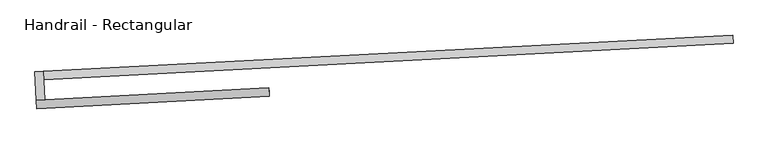
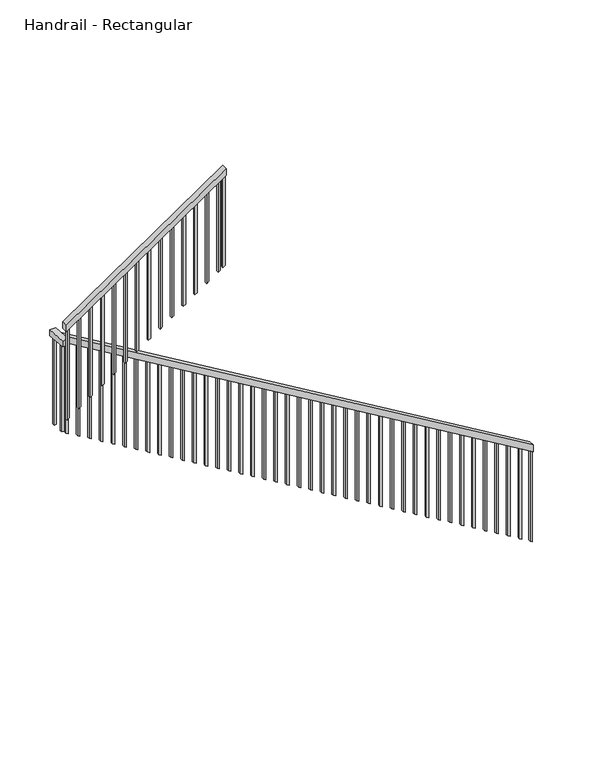
"""IFC4 building model written with IfcOpenShell, lengths in millimetres: railing geometry, Handrail - Rectangular."""

import ifcopenshell
import ifcopenshell.guid

model = None  # the IFC model being written
_history = None  # IfcOwnerHistory: only IFC2X3 demands one
_inside = {}  # id of a spatial element -> (the spatial element, [elements in it])
_under = {}  # id of a project, library or spatial element -> (it, [spatial elements below it])
_declared = {}  # id of a project -> (the project, [libraries it declares])
_typed = {}  # id of a type object -> (the type object, [elements of that type])
_made_of = {}  # id of a material, layer set ... -> (it, [elements and type objects made of it])


def new_model(schema):
    """Start an empty IFC model of exactly this schema.

    Asked for "IFC4X3", IfcOpenShell would pick the latest addendum, in which some entities
    have other attributes; the version numbers below select the first issue.
    IFC2X3 requires an IfcOwnerHistory on every rooted entity: one is made here for all.
    """
    global model, _history
    if schema == "IFC4X3":
        model = ifcopenshell.file(schema_version=(4, 3, 0, 0))
    else:
        model = ifcopenshell.file(schema=schema)
    _inside.clear()
    _under.clear()
    _declared.clear()
    _typed.clear()
    _made_of.clear()
    _history = None
    if model.schema == "IFC2X3":
        org = make("IfcOrganization", Name="unknown")
        user = make(
            "IfcPersonAndOrganization",
            ThePerson=make("IfcPerson", FamilyName="unknown"),
            TheOrganization=org,
        )
        app = make(
            "IfcApplication",
            ApplicationDeveloper=org,
            Version="unknown",
            ApplicationFullName="unknown",
            ApplicationIdentifier="unknown",
        )
        _history = make(
            "IfcOwnerHistory",
            OwningUser=user,
            OwningApplication=app,
            ChangeAction="ADDED",
            CreationDate=0,
        )
    return model


def make(cls, **values):
    """One entity of the class cls with the attributes given. An attribute that is None is left unset."""
    return model.create_entity(
        cls, **{name: value for name, value in values.items() if value is not None}
    )


def rooted(cls, **values):
    """An entity with a GlobalId (a new one), such as an element, a storey or a relation."""
    return make(cls, GlobalId=ifcopenshell.guid.new(), OwnerHistory=_history, **values)


def si_unit(unit_type, name, prefix=None):
    """IfcSIUnit, for example si_unit("LENGTHUNIT", "METRE", prefix="MILLI")."""
    return make("IfcSIUnit", UnitType=unit_type, Prefix=prefix, Name=name)


def assignment(units):
    """IfcUnitAssignment: the units of a project."""
    return None if units is None else make("IfcUnitAssignment", Units=units)


def point(xyz):
    """IfcCartesianPoint."""
    return None if xyz is None else make("IfcCartesianPoint", Coordinates=xyz)


def direction(xyz):
    """IfcDirection."""
    return None if xyz is None else make("IfcDirection", DirectionRatios=xyz)


def frame(location, z_axis=None, x_axis=None):
    """IfcAxis2Placement3D, a coordinate frame: its origin and axes. An axis left out is left unset."""
    return make(
        "IfcAxis2Placement3D",
        Location=point(location),
        Axis=direction(z_axis),
        RefDirection=direction(x_axis),
    )


def origin():
    """The frame at (0, 0, 0) with its axes left unset."""
    return frame((0.0, 0.0, 0.0))


def place(relative_to, where):
    """IfcLocalPlacement: puts the frame where relative to a parent placement (None: the world)."""
    return make(
        "IfcLocalPlacement", PlacementRelTo=relative_to, RelativePlacement=where
    )


def context(
    kind, dimensions, precision=None, world=None, true_north=None, identifier=None
):
    """IfcGeometricRepresentationContext, for example the 3D "Model" context."""
    return make(
        "IfcGeometricRepresentationContext",
        ContextIdentifier=identifier,
        ContextType=kind,
        CoordinateSpaceDimension=dimensions,
        Precision=precision,
        WorldCoordinateSystem=world,
        TrueNorth=true_north,
    )


def project(units=None, contexts=None):
    """IfcProject with its units and contexts."""
    return rooted(
        "IfcProject",
        Name="project",
        RepresentationContexts=contexts,
        UnitsInContext=assignment(units),
    )


def spatial(cls, under=None, at=None, **own):
    """A site, building, storey or space (cls), placed at a placement, below another one or the project."""
    s = rooted(cls, ObjectPlacement=at, **own)
    if under is not None:
        _under.setdefault(under.id(), (under, []))[1].append(s)
    return s


def polyline(points):
    """IfcPolyline through the points."""
    return make("IfcPolyline", Points=[point(p) for p in points])


def outline(outer, holes=None, kind="AREA"):
    """IfcArbitraryClosedProfileDef: a profile drawn as a closed curve; with holes, ...WithVoids."""
    if holes is None:
        return make("IfcArbitraryClosedProfileDef", ProfileType=kind, OuterCurve=outer)
    return make(
        "IfcArbitraryProfileDefWithVoids",
        ProfileType=kind,
        OuterCurve=outer,
        InnerCurves=holes,
    )


def extrude(swept, where, along, depth):
    """IfcExtrudedAreaSolid: the profile swept, set in the frame where, extruded along a direction by depth."""
    return make(
        "IfcExtrudedAreaSolid",
        SweptArea=swept,
        Position=where,
        ExtrudedDirection=direction(along),
        Depth=depth,
    )


def shape(context_of_items, identifier, shape_type, items):
    """IfcShapeRepresentation: the items that make up one representation, for example the "Body"."""
    return make(
        "IfcShapeRepresentation",
        ContextOfItems=context_of_items,
        RepresentationIdentifier=identifier,
        RepresentationType=shape_type,
        Items=items,
    )


def source(mapping_origin, context_of_items, identifier, shape_type, items):
    """IfcRepresentationMap: a shape defined once, which mapped items show again and again."""
    return make(
        "IfcRepresentationMap",
        MappingOrigin=mapping_origin,
        MappedRepresentation=shape(context_of_items, identifier, shape_type, items),
    )


def transform(
    local_origin,
    x_axis=None,
    y_axis=None,
    z_axis=None,
    scale=None,
    scale2=None,
    scale3=None,
    uniform=True,
):
    """IfcCartesianTransformationOperator3D, or its non-uniform kind. x_axis, y_axis, z_axis: its Axis1, 2, 3."""
    if uniform:
        return make(
            "IfcCartesianTransformationOperator3D",
            Axis1=direction(x_axis),
            Axis2=direction(y_axis),
            LocalOrigin=point(local_origin),
            Scale=scale,
            Axis3=direction(z_axis),
        )
    return make(
        "IfcCartesianTransformationOperator3DnonUniform",
        Axis1=direction(x_axis),
        Axis2=direction(y_axis),
        LocalOrigin=point(local_origin),
        Scale=scale,
        Axis3=direction(z_axis),
        Scale2=scale2,
        Scale3=scale3,
    )


def mapped(mapping_source, mapping_target):
    """IfcMappedItem: shows the shape of a source again, moved by a transform."""
    return make(
        "IfcMappedItem", MappingSource=mapping_source, MappingTarget=mapping_target
    )


def made_of(thing, what):
    """Note that an element or type object is made of a material, layer set ...; save() writes the relation."""
    if what is not None:
        _made_of.setdefault(what.id(), (what, []))[1].append(thing)
    return thing


def element(
    cls,
    number,
    at=None,
    inside=None,
    cuts=None,
    type_object=None,
    material=None,
    context=None,
    identifier="Body",
    shape_type=None,
    held_by="IfcProductDefinitionShape",
    body=None,
    shapes=None,
    **own,
):
    """One element of the class cls, such as IfcWall. Its Tag is "e" and its number.

    at: its placement. inside: the storey or other place that contains it. cuts: it is an
    opening in that element (IfcRelVoidsElement). A single representation is given by context,
    identifier, shape_type and body (its items); several are given by shapes. held_by: the class
    of the entity that holds the representations. save() writes the other relations.
    """
    e = rooted(cls, Tag="e%d" % number, ObjectPlacement=at, **own)
    if body is not None:
        shapes = [shape(context, identifier, shape_type, body)]
    if shapes is not None:
        e.Representation = make(held_by, Representations=shapes)
    if inside is not None:
        _inside.setdefault(inside.id(), (inside, []))[1].append(e)
    if cuts is not None:
        rooted(
            "IfcRelVoidsElement", RelatingBuildingElement=cuts, RelatedOpeningElement=e
        )
    if type_object is not None:
        _typed.setdefault(type_object.id(), (type_object, []))[1].append(e)
    return made_of(e, material)


def aggregate(whole, parts):
    """IfcRelAggregates: a whole, such as a stair, and the parts it consists of."""
    return rooted("IfcRelAggregates", RelatingObject=whole, RelatedObjects=parts)


def save(model, path):
    """Write the relations noted so far, then the file.

    IfcRelAggregates (storeys below a building ...), IfcRelContainedInSpatialStructure (elements
    in a storey), IfcRelDefinesByType, IfcRelAssociatesMaterial and IfcRelDeclares: one each for
    every whole, place, type object, material and project.
    """
    for whole, parts in _under.values():
        aggregate(whole, parts)
    for where, things in _inside.values():
        rooted(
            "IfcRelContainedInSpatialStructure",
            RelatedElements=things,
            RelatingStructure=where,
        )
    for kind, things in _typed.values():
        rooted("IfcRelDefinesByType", RelatedObjects=things, RelatingType=kind)
    for what, things in _made_of.values():
        rooted("IfcRelAssociatesMaterial", RelatedObjects=things, RelatingMaterial=what)
    for by, libraries in _declared.values():
        rooted("IfcRelDeclares", RelatingContext=by, RelatedDefinitions=libraries)
    model.write(path)


def handrail_rectangular_b2c7f8ce(model_context):
    return source(origin(), model_context, "Body", "SweptSolid", [
        extrude(outline(polyline([(-31.4876033, -50.8), (0.0, 0.0), (4871.0206406, 0.0), (4839.5330373, -50.8), (-31.4876033, -50.8)])), frame((12083.9919851, -25001.0309623, 1087.5818182), z_axis=(-0.05233595624293972, 0.9986295347545743, 0.0), x_axis=(-0.8488007555029385, -0.04448376264967305, 0.5268381841876767)), (0.0, 0.0, 1.0), 50.8),
        extrude(outline(polyline([(7896.0769384, -25169.6405746), (7946.8073187, -25166.981908), (7955.7803184, -25338.1969417), (7905.0499381, -25340.8556083), (7896.0769384, -25169.6405746)])), frame((0.0, 0.0, 3634.5090909), z_axis=(0.0, 0.0, 1.0), x_axis=(1.0, 0.0, 0.0)), (0.0, 0.0, 1.0), 50.8),
        extrude(outline(polyline([(31.4876033, -50.8), (0.0, 0.0), (1643.5959216, 0.0), (1675.0835249, -50.8), (31.4876033, -50.8)])), frame((7907.7086047, -25391.5859887, 3798.7237847), z_axis=(-0.052335956242938755, 0.9986295347545742, 0.0), x_axis=(0.8488007555029388, 0.044483762649671764, 0.5268381841876766)), (0.0, 0.0, 1.0), 50.8),
        extrude(outline(polyline([(234.5039256, 19.0500001), (1048.9045305, 19.0500001), (1037.0966792, 0.0), (222.6960744, 0.0), (234.5039256, 19.0500001)])), frame((9260.7447974, -25304.7795805, 4861.7452723), z_axis=(-0.052335956242940136, 0.9986295347545743, 0.0), x_axis=(0.0, 0.0, -1.0)), (0.0, 0.0, 1.0), 19.05),
        extrude(outline(polyline([(234.5039257, 19.05), (1048.9045305, 19.05), (1037.0966792, 0.0), (222.6960744, 0.0), (234.5039257, 19.05)])), frame((9159.2840366, -25310.0969137, 4798.7700657), z_axis=(-0.052335956242940136, 0.9986295347545743, 0.0), x_axis=(0.0, 0.0, -1.0)), (0.0, 0.0, 1.0), 19.05),
        extrude(outline(polyline([(234.5039256, 19.05), (1048.9045304, 19.05), (1037.0966791, 0.0), (222.6960743, 0.0), (234.5039256, 19.05)])), frame((9057.8232759, -25315.4142468, 4735.794859), z_axis=(-0.052335956242940136, 0.9986295347545743, 0.0), x_axis=(0.0, 0.0, -1.0)), (0.0, 0.0, 1.0), 19.05),
        extrude(outline(polyline([(234.5039256, 19.0500001), (1048.9045304, 19.0500001), (1037.0966792, 0.0), (222.6960743, 0.0), (234.5039256, 19.0500001)])), frame((8956.3625152, -25320.73158, 4672.8196524), z_axis=(-0.052335956242940136, 0.9986295347545743, 0.0), x_axis=(0.0, 0.0, -1.0)), (0.0, 0.0, 1.0), 19.05),
        extrude(outline(polyline([(234.5039256, 19.05), (1048.9045304, 19.05), (1037.0966792, 0.0), (222.6960744, 0.0), (234.5039256, 19.05)])), frame((8854.9017544, -25326.0489131, 4609.8444458), z_axis=(-0.052335956242940136, 0.9986295347545743, 0.0), x_axis=(0.0, 0.0, -1.0)), (0.0, 0.0, 1.0), 19.05),
        extrude(outline(polyline([(234.5039256, 19.05), (1048.9045304, 19.05), (1037.0966792, 0.0), (222.6960744, 0.0), (234.5039256, 19.05)])), frame((8753.4409937, -25331.3662463, 4546.8692392), z_axis=(-0.052335956242940136, 0.9986295347545743, 0.0), x_axis=(0.0, 0.0, -1.0)), (0.0, 0.0, 1.0), 19.05),
        extrude(outline(polyline([(234.5039256, 19.0500001), (1048.9045304, 19.0500001), (1037.0966792, 0.0), (222.6960744, 0.0), (234.5039256, 19.0500001)])), frame((8651.980233, -25336.6835795, 4483.8940326), z_axis=(-0.052335956242940136, 0.9986295347545743, 0.0), x_axis=(0.0, 0.0, -1.0)), (0.0, 0.0, 1.0), 19.05),
        extrude(outline(polyline([(234.5039256, 19.05), (1048.9045304, 19.05), (1037.0966792, 0.0), (222.6960744, 0.0), (234.5039256, 19.05)])), frame((8550.5194722, -25342.0009126, 4420.918826), z_axis=(-0.052335956242940136, 0.9986295347545743, 0.0), x_axis=(0.0, 0.0, -1.0)), (0.0, 0.0, 1.0), 19.05),
        extrude(outline(polyline([(234.5039256, 19.05), (1048.9045305, 19.05), (1037.0966792, 0.0), (222.6960744, 0.0), (234.5039256, 19.05)])), frame((8449.0587115, -25347.3182458, 4357.9436194), z_axis=(-0.052335956242940136, 0.9986295347545743, 0.0), x_axis=(0.0, 0.0, -1.0)), (0.0, 0.0, 1.0), 19.05),
        extrude(outline(polyline([(234.5039257, 19.0500001), (1048.9045305, 19.0500001), (1037.0966792, 0.0), (222.6960744, 0.0), (234.5039257, 19.0500001)])), frame((8347.5979508, -25352.6355789, 4294.9684128), z_axis=(-0.052335956242940136, 0.9986295347545743, 0.0), x_axis=(0.0, 0.0, -1.0)), (0.0, 0.0, 1.0), 19.05),
        extrude(outline(polyline([(234.5039257, 19.05), (1048.9045305, 19.05), (1037.0966792, 0.0), (222.6960744, 0.0), (234.5039257, 19.05)])), frame((8246.13719, -25357.9529121, 4231.9932062), z_axis=(-0.052335956242940136, 0.9986295347545743, 0.0), x_axis=(0.0, 0.0, -1.0)), (0.0, 0.0, 1.0), 19.05),
        extrude(outline(polyline([(234.5039256, 19.05), (1048.9045304, 19.05), (1037.0966791, 0.0), (222.6960743, 0.0), (234.5039256, 19.05)])), frame((8144.6764293, -25363.2702452, 4169.0179995), z_axis=(-0.052335956242940136, 0.9986295347545743, 0.0), x_axis=(0.0, 0.0, -1.0)), (0.0, 0.0, 1.0), 19.05),
        extrude(outline(polyline([(234.5039256, 19.0500001), (1048.9045304, 19.0500001), (1037.0966792, 0.0), (222.6960743, 0.0), (234.5039256, 19.0500001)])), frame((8043.2156686, -25368.5875784, 4106.0427929), z_axis=(-0.052335956242940136, 0.9986295347545743, 0.0), x_axis=(0.0, 0.0, -1.0)), (0.0, 0.0, 1.0), 19.05),
        extrude(outline(polyline([(7937.1022413, -25285.1267459), (7938.0992413, -25304.1506385), (7919.0753487, -25305.1476385), (7918.0783487, -25286.1237459), (7937.1022413, -25285.1267459)])), frame((0.0, 0.0, 2847.1090909), z_axis=(0.0, 0.0, 1.0), x_axis=(1.0, 0.0, 0.0)), (0.0, 0.0, 1.0), 787.4),
        extrude(outline(polyline([(222.6960744, 19.0500001), (1037.0966792, 19.0500001), (1048.9045304, 0.0), (234.5039256, 0.0), (222.6960744, 19.0500001)])), frame((8034.2426689, -25197.3725446, 3775.4229582), z_axis=(-0.05233595624293971, 0.9986295347545743, 0.0), x_axis=(0.0, 0.0, -1.0)), (0.0, 0.0, 1.0), 19.05),
        extrude(outline(polyline([(222.6960744, 19.05), (1037.0966792, 19.05), (1048.9045304, 0.0), (234.5039256, 0.0), (222.6960744, 19.05)])), frame((8135.7034296, -25192.0552115, 3712.4477516), z_axis=(-0.05233595624293971, 0.9986295347545743, 0.0), x_axis=(0.0, 0.0, -1.0)), (0.0, 0.0, 1.0), 19.05),
        extrude(outline(polyline([(222.6960744, 19.05), (1037.0966792, 19.05), (1048.9045304, 0.0), (234.5039256, 0.0), (222.6960744, 19.05)])), frame((8237.1641903, -25186.7378783, 3649.472545), z_axis=(-0.05233595624293971, 0.9986295347545743, 0.0), x_axis=(0.0, 0.0, -1.0)), (0.0, 0.0, 1.0), 19.05),
        extrude(outline(polyline([(222.6960744, 19.0500001), (1037.0966792, 19.0500001), (1048.9045304, 0.0), (234.5039256, 0.0), (222.6960744, 19.0500001)])), frame((8338.6249511, -25181.4205452, 3586.4973384), z_axis=(-0.05233595624293971, 0.9986295347545743, 0.0), x_axis=(0.0, 0.0, -1.0)), (0.0, 0.0, 1.0), 19.05),
        extrude(outline(polyline([(222.6960744, 19.05), (1037.0966792, 19.05), (1048.9045305, 0.0), (234.5039256, 0.0), (222.6960744, 19.05)])), frame((8440.0857118, -25176.103212, 3523.5221318), z_axis=(-0.05233595624293971, 0.9986295347545743, 0.0), x_axis=(0.0, 0.0, -1.0)), (0.0, 0.0, 1.0), 19.05),
        extrude(outline(polyline([(222.6960744, 19.05), (1037.0966792, 19.05), (1048.9045305, 0.0), (234.5039257, 0.0), (222.6960744, 19.05)])), frame((8541.5464725, -25170.7858789, 3460.5469252), z_axis=(-0.05233595624293971, 0.9986295347545743, 0.0), x_axis=(0.0, 0.0, -1.0)), (0.0, 0.0, 1.0), 19.05),
        extrude(outline(polyline([(222.6960744, 19.0500001), (1037.0966792, 19.0500001), (1048.9045305, 0.0), (234.5039257, 0.0), (222.6960744, 19.0500001)])), frame((8643.0072333, -25165.4685457, 3397.5717186), z_axis=(-0.05233595624293971, 0.9986295347545743, 0.0), x_axis=(0.0, 0.0, -1.0)), (0.0, 0.0, 1.0), 19.05),
        extrude(outline(polyline([(222.6960743, 19.05), (1037.0966791, 19.05), (1048.9045304, 0.0), (234.5039256, 0.0), (222.6960743, 19.05)])), frame((8744.467994, -25160.1512126, 3334.5965119), z_axis=(-0.05233595624293971, 0.9986295347545743, 0.0), x_axis=(0.0, 0.0, -1.0)), (0.0, 0.0, 1.0), 19.05),
        extrude(outline(polyline([(222.6960744, 19.05), (1037.0966792, 19.05), (1048.9045304, 0.0), (234.5039256, 0.0), (222.6960744, 19.05)])), frame((8845.9287547, -25154.8338794, 3271.6213053), z_axis=(-0.05233595624293971, 0.9986295347545743, 0.0), x_axis=(0.0, 0.0, -1.0)), (0.0, 0.0, 1.0), 19.05),
        extrude(outline(polyline([(222.6960744, 19.0500001), (1037.0966792, 19.0500001), (1048.9045304, 0.0), (234.5039256, 0.0), (222.6960744, 19.0500001)])), frame((8947.3895155, -25149.5165463, 3208.6460987), z_axis=(-0.05233595624293971, 0.9986295347545743, 0.0), x_axis=(0.0, 0.0, -1.0)), (0.0, 0.0, 1.0), 19.05),
        extrude(outline(polyline([(222.6960744, 19.05), (1037.0966792, 19.05), (1048.9045304, 0.0), (234.5039256, 0.0), (222.6960744, 19.05)])), frame((9048.8502762, -25144.1992131, 3145.6708921), z_axis=(-0.05233595624293971, 0.9986295347545743, 0.0), x_axis=(0.0, 0.0, -1.0)), (0.0, 0.0, 1.0), 19.05),
        extrude(outline(polyline([(222.6960744, 19.05), (1037.0966792, 19.05), (1048.9045304, 0.0), (234.5039256, 0.0), (222.6960744, 19.05)])), frame((9150.3110369, -25138.8818799, 3082.6956855), z_axis=(-0.05233595624293971, 0.9986295347545743, 0.0), x_axis=(0.0, 0.0, -1.0)), (0.0, 0.0, 1.0), 19.05),
        extrude(outline(polyline([(222.6960744, 19.0500001), (1037.0966792, 19.0500001), (1048.9045304, 0.0), (234.5039256, 0.0), (222.6960744, 19.0500001)])), frame((9251.7717977, -25133.5645468, 3019.7204789), z_axis=(-0.05233595624293971, 0.9986295347545743, 0.0), x_axis=(0.0, 0.0, -1.0)), (0.0, 0.0, 1.0), 19.05),
        extrude(outline(polyline([(222.6960744, 19.05), (1037.0966792, 19.05), (1048.9045305, 0.0), (234.5039256, 0.0), (222.6960744, 19.05)])), frame((9353.2325584, -25128.2472136, 2956.7452723), z_axis=(-0.05233595624293971, 0.9986295347545743, 0.0), x_axis=(0.0, 0.0, -1.0)), (0.0, 0.0, 1.0), 19.05),
        extrude(outline(polyline([(222.6960744, 19.05), (1037.0966792, 19.05), (1048.9045305, 0.0), (234.5039257, 0.0), (222.6960744, 19.05)])), frame((9454.6933191, -25122.9298805, 2893.7700657), z_axis=(-0.05233595624293971, 0.9986295347545743, 0.0), x_axis=(0.0, 0.0, -1.0)), (0.0, 0.0, 1.0), 19.05),
        extrude(outline(polyline([(222.6960743, 19.05), (1037.0966791, 19.05), (1048.9045304, 0.0), (234.5039256, 0.0), (222.6960743, 19.05)])), frame((9556.1540798, -25117.6125473, 2830.794859), z_axis=(-0.05233595624293971, 0.9986295347545743, 0.0), x_axis=(0.0, 0.0, -1.0)), (0.0, 0.0, 1.0), 19.05),
        extrude(outline(polyline([(222.6960743, 19.0500001), (1037.0966792, 19.0500001), (1048.9045304, 0.0), (234.5039256, 0.0), (222.6960743, 19.0500001)])), frame((9657.6148406, -25112.2952142, 2767.8196524), z_axis=(-0.05233595624293971, 0.9986295347545743, 0.0), x_axis=(0.0, 0.0, -1.0)), (0.0, 0.0, 1.0), 19.05),
        extrude(outline(polyline([(222.6960744, 19.05), (1037.0966792, 19.05), (1048.9045304, 0.0), (234.5039256, 0.0), (222.6960744, 19.05)])), frame((9759.0756013, -25106.977881, 2704.8444458), z_axis=(-0.05233595624293971, 0.9986295347545743, 0.0), x_axis=(0.0, 0.0, -1.0)), (0.0, 0.0, 1.0), 19.05),
        extrude(outline(polyline([(222.6960744, 19.05), (1037.0966792, 19.05), (1048.9045304, 0.0), (234.5039256, 0.0), (222.6960744, 19.05)])), frame((9860.536362, -25101.6605479, 2641.8692392), z_axis=(-0.05233595624293971, 0.9986295347545743, 0.0), x_axis=(0.0, 0.0, -1.0)), (0.0, 0.0, 1.0), 19.05),
        extrude(outline(polyline([(222.6960744, 19.0500001), (1037.0966792, 19.0500001), (1048.9045304, 0.0), (234.5039256, 0.0), (222.6960744, 19.0500001)])), frame((9961.9971228, -25096.3432147, 2578.8940326), z_axis=(-0.05233595624293971, 0.9986295347545743, 0.0), x_axis=(0.0, 0.0, -1.0)), (0.0, 0.0, 1.0), 19.05),
        extrude(outline(polyline([(222.6960744, 19.05), (1037.0966792, 19.05), (1048.9045304, 0.0), (234.5039256, 0.0), (222.6960744, 19.05)])), frame((10063.4578835, -25091.0258816, 2515.918826), z_axis=(-0.05233595624293971, 0.9986295347545743, 0.0), x_axis=(0.0, 0.0, -1.0)), (0.0, 0.0, 1.0), 19.05),
        extrude(outline(polyline([(222.6960744, 19.05), (1037.0966792, 19.05), (1048.9045305, 0.0), (234.5039256, 0.0), (222.6960744, 19.05)])), frame((10164.9186442, -25085.7085484, 2452.9436194), z_axis=(-0.05233595624293971, 0.9986295347545743, 0.0), x_axis=(0.0, 0.0, -1.0)), (0.0, 0.0, 1.0), 19.05),
        extrude(outline(polyline([(222.6960744, 19.0500001), (1037.0966792, 19.0500001), (1048.9045305, 0.0), (234.5039257, 0.0), (222.6960744, 19.0500001)])), frame((10266.379405, -25080.3912153, 2389.9684128), z_axis=(-0.05233595624293971, 0.9986295347545743, 0.0), x_axis=(0.0, 0.0, -1.0)), (0.0, 0.0, 1.0), 19.05),
        extrude(outline(polyline([(222.6960744, 19.05), (1037.0966792, 19.05), (1048.9045305, 0.0), (234.5039257, 0.0), (222.6960744, 19.05)])), frame((10367.8401657, -25075.0738821, 2326.9932062), z_axis=(-0.05233595624293971, 0.9986295347545743, 0.0), x_axis=(0.0, 0.0, -1.0)), (0.0, 0.0, 1.0), 19.05),
        extrude(outline(polyline([(222.6960743, 19.05), (1037.0966791, 19.05), (1048.9045304, 0.0), (234.5039256, 0.0), (222.6960743, 19.05)])), frame((10469.3009264, -25069.7565489, 2264.0179995), z_axis=(-0.05233595624293971, 0.9986295347545743, 0.0), x_axis=(0.0, 0.0, -1.0)), (0.0, 0.0, 1.0), 19.05),
        extrude(outline(polyline([(222.6960743, 19.0500001), (1037.0966792, 19.0500001), (1048.9045304, 0.0), (234.5039256, 0.0), (222.6960743, 19.0500001)])), frame((10570.7616872, -25064.4392158, 2201.0427929), z_axis=(-0.05233595624293971, 0.9986295347545743, 0.0), x_axis=(0.0, 0.0, -1.0)), (0.0, 0.0, 1.0), 19.05),
        extrude(outline(polyline([(222.6960744, 19.05), (1037.0966792, 19.05), (1048.9045304, 0.0), (234.5039256, 0.0), (222.6960744, 19.05)])), frame((10672.2224479, -25059.1218826, 2138.0675863), z_axis=(-0.05233595624293971, 0.9986295347545743, 0.0), x_axis=(0.0, 0.0, -1.0)), (0.0, 0.0, 1.0), 19.05),
        extrude(outline(polyline([(222.6960744, 19.05), (1037.0966792, 19.05), (1048.9045304, 0.0), (234.5039256, 0.0), (222.6960744, 19.05)])), frame((10773.6832086, -25053.8045495, 2075.0923797), z_axis=(-0.05233595624293971, 0.9986295347545743, 0.0), x_axis=(0.0, 0.0, -1.0)), (0.0, 0.0, 1.0), 19.05),
        extrude(outline(polyline([(222.6960744, 19.0500001), (1037.0966792, 19.0500001), (1048.9045304, 0.0), (234.5039256, 0.0), (222.6960744, 19.0500001)])), frame((10875.1439694, -25048.4872163, 2012.1171731), z_axis=(-0.05233595624293971, 0.9986295347545743, 0.0), x_axis=(0.0, 0.0, -1.0)), (0.0, 0.0, 1.0), 19.05),
        extrude(outline(polyline([(222.6960744, 19.0500001), (1037.0966792, 19.0500001), (1048.9045304, 0.0), (234.5039256, 0.0), (222.6960744, 19.0500001)])), frame((10976.6047301, -25043.1698832, 1949.1419665), z_axis=(-0.05233595624293971, 0.9986295347545743, 0.0), x_axis=(0.0, 0.0, -1.0)), (0.0, 0.0, 1.0), 19.05),
        extrude(outline(polyline([(222.6960744, 19.05), (1037.0966792, 19.05), (1048.9045305, 0.0), (234.5039256, 0.0), (222.6960744, 19.05)])), frame((11078.0654908, -25037.85255, 1886.1667599), z_axis=(-0.05233595624293971, 0.9986295347545743, 0.0), x_axis=(0.0, 0.0, -1.0)), (0.0, 0.0, 1.0), 19.05),
        extrude(outline(polyline([(222.6960744, 19.05), (1037.0966792, 19.05), (1048.9045305, 0.0), (234.5039257, 0.0), (222.6960744, 19.05)])), frame((11179.5262515, -25032.5352169, 1823.1915533), z_axis=(-0.05233595624293971, 0.9986295347545743, 0.0), x_axis=(0.0, 0.0, -1.0)), (0.0, 0.0, 1.0), 19.05),
        extrude(outline(polyline([(222.6960744, 19.0500001), (1037.0966792, 19.0500001), (1048.9045305, 0.0), (234.5039257, 0.0), (222.6960744, 19.0500001)])), frame((11280.9870123, -25027.2178837, 1760.2163467), z_axis=(-0.05233595624293971, 0.9986295347545743, 0.0), x_axis=(0.0, 0.0, -1.0)), (0.0, 0.0, 1.0), 19.05),
        extrude(outline(polyline([(222.6960743, 19.05), (1037.0966792, 19.05), (1048.9045304, 0.0), (234.5039256, 0.0), (222.6960743, 19.05)])), frame((11382.447773, -25021.9005506, 1697.24114), z_axis=(-0.05233595624293971, 0.9986295347545743, 0.0), x_axis=(0.0, 0.0, -1.0)), (0.0, 0.0, 1.0), 19.05),
        extrude(outline(polyline([(222.6960744, 19.05), (1037.0966792, 19.05), (1048.9045304, 0.0), (234.5039256, 0.0), (222.6960744, 19.05)])), frame((11483.9085337, -25016.5832174, 1634.2659334), z_axis=(-0.05233595624293971, 0.9986295347545743, 0.0), x_axis=(0.0, 0.0, -1.0)), (0.0, 0.0, 1.0), 19.05),
        extrude(outline(polyline([(222.6960744, 19.0500001), (1037.0966792, 19.0500001), (1048.9045304, 0.0), (234.5039256, 0.0), (222.6960744, 19.0500001)])), frame((11585.3692945, -25011.2658842, 1571.2907268), z_axis=(-0.05233595624293971, 0.9986295347545743, 0.0), x_axis=(0.0, 0.0, -1.0)), (0.0, 0.0, 1.0), 19.05),
        extrude(outline(polyline([(222.6960744, 19.05), (1037.0966792, 19.05), (1048.9045304, 0.0), (234.5039256, 0.0), (222.6960744, 19.05)])), frame((11686.8300552, -25005.9485511, 1508.3155202), z_axis=(-0.05233595624293971, 0.9986295347545743, 0.0), x_axis=(0.0, 0.0, -1.0)), (0.0, 0.0, 1.0), 19.05),
        extrude(outline(polyline([(222.6960744, 19.05), (1037.0966792, 19.05), (1048.9045304, 0.0), (234.5039256, 0.0), (222.6960744, 19.05)])), frame((11788.2908159, -25000.6312179, 1445.3403136), z_axis=(-0.05233595624293971, 0.9986295347545743, 0.0), x_axis=(0.0, 0.0, -1.0)), (0.0, 0.0, 1.0), 19.05),
        extrude(outline(polyline([(222.6960744, 19.0500001), (1037.0966792, 19.0500001), (1048.9045304, 0.0), (234.5039256, 0.0), (222.6960744, 19.0500001)])), frame((11889.7515767, -24995.3138848, 1382.365107), z_axis=(-0.05233595624293971, 0.9986295347545743, 0.0), x_axis=(0.0, 0.0, -1.0)), (0.0, 0.0, 1.0), 19.05),
        extrude(outline(polyline([(222.6960744, 19.05), (1037.0966792, 19.05), (1048.9045305, 0.0), (234.5039257, 0.0), (222.6960744, 19.05)])), frame((11991.2123374, -24989.9965516, 1319.3899004), z_axis=(-0.05233595624293971, 0.9986295347545743, 0.0), x_axis=(0.0, 0.0, -1.0)), (0.0, 0.0, 1.0), 19.05),
        extrude(outline(polyline([(234.5039256, 19.0500001), (1048.9045304, 19.0500001), (1037.0966792, 0.0), (222.6960744, 0.0), (234.5039256, 19.0500001)])), frame((7941.7549079, -25373.9049115, 4043.0675863), z_axis=(-0.052335956242940136, 0.9986295347545743, 0.0), x_axis=(0.0, 0.0, -1.0)), (0.0, 0.0, 1.0), 19.05),
        extrude(outline(polyline([(7931.7849082, -25183.6659852), (7932.7819082, -25202.6898778), (7913.7580155, -25203.6868778), (7912.7610155, -25184.6629851), (7931.7849082, -25183.6659852)])), frame((0.0, 0.0, 2847.1090909), z_axis=(0.0, 0.0, 1.0), x_axis=(1.0, 0.0, 0.0)), (0.0, 0.0, 1.0), 787.4),
        extrude(outline(polyline([(234.5039257, 19.05), (1048.9045305, 19.05), (1037.0966792, 0.0), (222.6960744, 0.0), (234.5039257, 19.05)])), frame((9301.9632314, -25302.6194139, 4887.32895), z_axis=(-0.052335956242940136, 0.9986295347545743, 0.0), x_axis=(0.0, 0.0, -1.0)), (0.0, 0.0, 1.0), 19.05),
        extrude(outline(polyline([(222.6960744, 19.05), (1037.0966792, 19.05), (1048.9045305, 0.0), (234.5039256, 0.0), (222.6960744, 19.05)])), frame((12083.1611518, -24985.1777185, 1262.3186194), z_axis=(-0.05233595624293971, 0.9986295347545743, 0.0), x_axis=(0.0, 0.0, -1.0)), (0.0, 0.0, 1.0), 19.05),
    ])


if __name__ == "__main__":
    model = new_model("IFC4")
    model_context = context("Model", 3, world=origin())
    ifc_project = project(units=[si_unit("LENGTHUNIT", "METRE", prefix="MILLI")], contexts=[model_context])
    site = spatial("IfcSite", under=ifc_project)
    building = spatial("IfcBuilding", under=site)
    placement = place(None, origin())
    handrail_rectangular_shape = handrail_rectangular_b2c7f8ce(model_context)
    element("IfcRailing", 1, ObjectType="Handrail - Rectangular", at=placement, inside=building, context=model_context, shape_type="MappedRepresentation", body=[
        mapped(handrail_rectangular_shape, transform((0.0, 0.0, 0.0), x_axis=(1.0, 0.0, 0.0), y_axis=(0.0, 1.0, 0.0), z_axis=(0.0, 0.0, 1.0))),
    ])
    save(model, "model.ifc")
